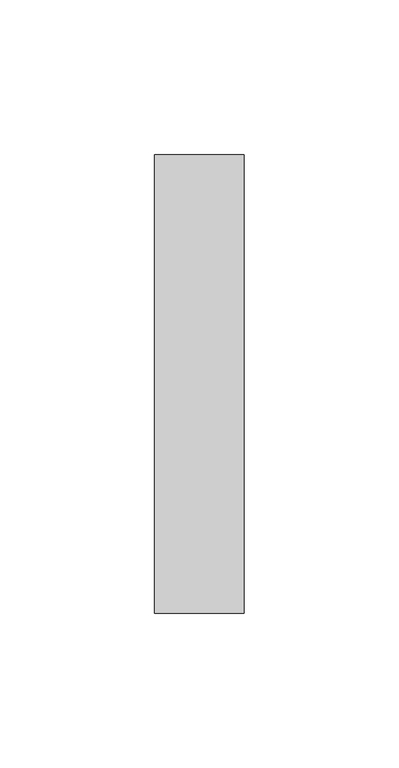
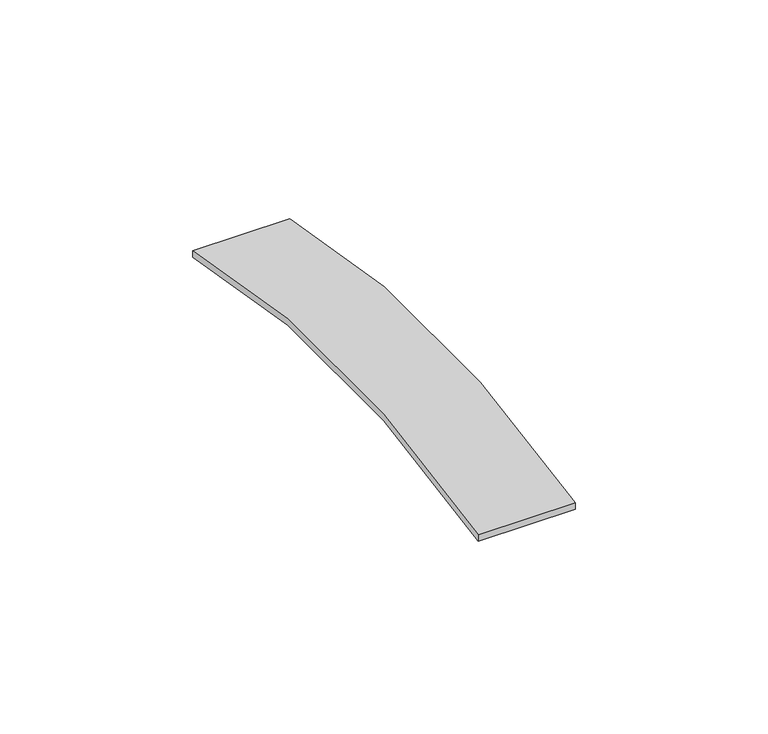
"""IFC4 building model written with IfcOpenShell, lengths in millimetres: proxy geometry, TN_ПВС 125-82_Защитная решетка : TN_ПВС 125-82_Защитная решетка."""

import ifcopenshell
import ifcopenshell.guid

model = None  # the IFC model being written
_history = None  # IfcOwnerHistory: only IFC2X3 demands one
_inside = {}  # id of a spatial element -> (the spatial element, [elements in it])
_under = {}  # id of a project, library or spatial element -> (it, [spatial elements below it])
_declared = {}  # id of a project -> (the project, [libraries it declares])
_typed = {}  # id of a type object -> (the type object, [elements of that type])
_made_of = {}  # id of a material, layer set ... -> (it, [elements and type objects made of it])


def new_model(schema):
    """Start an empty IFC model of exactly this schema.

    Asked for "IFC4X3", IfcOpenShell would pick the latest addendum, in which some entities
    have other attributes; the version numbers below select the first issue.
    IFC2X3 requires an IfcOwnerHistory on every rooted entity: one is made here for all.
    """
    global model, _history
    if schema == "IFC4X3":
        model = ifcopenshell.file(schema_version=(4, 3, 0, 0))
    else:
        model = ifcopenshell.file(schema=schema)
    _inside.clear()
    _under.clear()
    _declared.clear()
    _typed.clear()
    _made_of.clear()
    _history = None
    if model.schema == "IFC2X3":
        org = make("IfcOrganization", Name="unknown")
        user = make(
            "IfcPersonAndOrganization",
            ThePerson=make("IfcPerson", FamilyName="unknown"),
            TheOrganization=org,
        )
        app = make(
            "IfcApplication",
            ApplicationDeveloper=org,
            Version="unknown",
            ApplicationFullName="unknown",
            ApplicationIdentifier="unknown",
        )
        _history = make(
            "IfcOwnerHistory",
            OwningUser=user,
            OwningApplication=app,
            ChangeAction="ADDED",
            CreationDate=0,
        )
    return model


def make(cls, **values):
    """One entity of the class cls with the attributes given. An attribute that is None is left unset."""
    return model.create_entity(
        cls, **{name: value for name, value in values.items() if value is not None}
    )


def rooted(cls, **values):
    """An entity with a GlobalId (a new one), such as an element, a storey or a relation."""
    return make(cls, GlobalId=ifcopenshell.guid.new(), OwnerHistory=_history, **values)


def si_unit(unit_type, name, prefix=None):
    """IfcSIUnit, for example si_unit("LENGTHUNIT", "METRE", prefix="MILLI")."""
    return make("IfcSIUnit", UnitType=unit_type, Prefix=prefix, Name=name)


def assignment(units):
    """IfcUnitAssignment: the units of a project."""
    return None if units is None else make("IfcUnitAssignment", Units=units)


def point(xyz):
    """IfcCartesianPoint."""
    return None if xyz is None else make("IfcCartesianPoint", Coordinates=xyz)


def direction(xyz):
    """IfcDirection."""
    return None if xyz is None else make("IfcDirection", DirectionRatios=xyz)


def frame(location, z_axis=None, x_axis=None):
    """IfcAxis2Placement3D, a coordinate frame: its origin and axes. An axis left out is left unset."""
    return make(
        "IfcAxis2Placement3D",
        Location=point(location),
        Axis=direction(z_axis),
        RefDirection=direction(x_axis),
    )


def frame_2d(location, x_axis=None):
    """IfcAxis2Placement2D, a coordinate frame in the plane: its origin and x axis."""
    return make(
        "IfcAxis2Placement2D", Location=point(location), RefDirection=direction(x_axis)
    )


def origin():
    """The frame at (0, 0, 0) with its axes left unset."""
    return frame((0.0, 0.0, 0.0))


def place(relative_to, where):
    """IfcLocalPlacement: puts the frame where relative to a parent placement (None: the world)."""
    return make(
        "IfcLocalPlacement", PlacementRelTo=relative_to, RelativePlacement=where
    )


def context(
    kind, dimensions, precision=None, world=None, true_north=None, identifier=None
):
    """IfcGeometricRepresentationContext, for example the 3D "Model" context."""
    return make(
        "IfcGeometricRepresentationContext",
        ContextIdentifier=identifier,
        ContextType=kind,
        CoordinateSpaceDimension=dimensions,
        Precision=precision,
        WorldCoordinateSystem=world,
        TrueNorth=true_north,
    )


def project(units=None, contexts=None):
    """IfcProject with its units and contexts."""
    return rooted(
        "IfcProject",
        Name="project",
        RepresentationContexts=contexts,
        UnitsInContext=assignment(units),
    )


def spatial(cls, under=None, at=None, **own):
    """A site, building, storey or space (cls), placed at a placement, below another one or the project."""
    s = rooted(cls, ObjectPlacement=at, **own)
    if under is not None:
        _under.setdefault(under.id(), (under, []))[1].append(s)
    return s


def polyline(points):
    """IfcPolyline through the points."""
    return make("IfcPolyline", Points=[point(p) for p in points])


def circle_curve(where, radius):
    """IfcCircle in the frame where."""
    return make("IfcCircle", Position=where, Radius=radius)


def trimmed(basis, trim1, trim2, sense, master):
    """IfcTrimmedCurve: the piece of a basis curve between two trims."""
    return make(
        "IfcTrimmedCurve",
        BasisCurve=basis,
        Trim1=trim1,
        Trim2=trim2,
        SenseAgreement=sense,
        MasterRepresentation=master,
    )


def segment(curve, same_sense, transition):
    """IfcCompositeCurveSegment."""
    return make(
        "IfcCompositeCurveSegment",
        Transition=transition,
        SameSense=same_sense,
        ParentCurve=curve,
    )


def composite_curve(segments, self_intersect=None):
    """IfcCompositeCurve: segments joined end to end."""
    return make("IfcCompositeCurve", Segments=segments, SelfIntersect=self_intersect)


def outline(outer, holes=None, kind="AREA"):
    """IfcArbitraryClosedProfileDef: a profile drawn as a closed curve; with holes, ...WithVoids."""
    if holes is None:
        return make("IfcArbitraryClosedProfileDef", ProfileType=kind, OuterCurve=outer)
    return make(
        "IfcArbitraryProfileDefWithVoids",
        ProfileType=kind,
        OuterCurve=outer,
        InnerCurves=holes,
    )


def extrude(swept, where, along, depth):
    """IfcExtrudedAreaSolid: the profile swept, set in the frame where, extruded along a direction by depth."""
    return make(
        "IfcExtrudedAreaSolid",
        SweptArea=swept,
        Position=where,
        ExtrudedDirection=direction(along),
        Depth=depth,
    )


def shape(context_of_items, identifier, shape_type, items):
    """IfcShapeRepresentation: the items that make up one representation, for example the "Body"."""
    return make(
        "IfcShapeRepresentation",
        ContextOfItems=context_of_items,
        RepresentationIdentifier=identifier,
        RepresentationType=shape_type,
        Items=items,
    )


def source(mapping_origin, context_of_items, identifier, shape_type, items):
    """IfcRepresentationMap: a shape defined once, which mapped items show again and again."""
    return make(
        "IfcRepresentationMap",
        MappingOrigin=mapping_origin,
        MappedRepresentation=shape(context_of_items, identifier, shape_type, items),
    )


def transform(
    local_origin,
    x_axis=None,
    y_axis=None,
    z_axis=None,
    scale=None,
    scale2=None,
    scale3=None,
    uniform=True,
):
    """IfcCartesianTransformationOperator3D, or its non-uniform kind. x_axis, y_axis, z_axis: its Axis1, 2, 3."""
    if uniform:
        return make(
            "IfcCartesianTransformationOperator3D",
            Axis1=direction(x_axis),
            Axis2=direction(y_axis),
            LocalOrigin=point(local_origin),
            Scale=scale,
            Axis3=direction(z_axis),
        )
    return make(
        "IfcCartesianTransformationOperator3DnonUniform",
        Axis1=direction(x_axis),
        Axis2=direction(y_axis),
        LocalOrigin=point(local_origin),
        Scale=scale,
        Axis3=direction(z_axis),
        Scale2=scale2,
        Scale3=scale3,
    )


def mapped(mapping_source, mapping_target):
    """IfcMappedItem: shows the shape of a source again, moved by a transform."""
    return make(
        "IfcMappedItem", MappingSource=mapping_source, MappingTarget=mapping_target
    )


def made_of(thing, what):
    """Note that an element or type object is made of a material, layer set ...; save() writes the relation."""
    if what is not None:
        _made_of.setdefault(what.id(), (what, []))[1].append(thing)
    return thing


def element(
    cls,
    number,
    at=None,
    inside=None,
    cuts=None,
    type_object=None,
    material=None,
    context=None,
    identifier="Body",
    shape_type=None,
    held_by="IfcProductDefinitionShape",
    body=None,
    shapes=None,
    **own,
):
    """One element of the class cls, such as IfcWall. Its Tag is "e" and its number.

    at: its placement. inside: the storey or other place that contains it. cuts: it is an
    opening in that element (IfcRelVoidsElement). A single representation is given by context,
    identifier, shape_type and body (its items); several are given by shapes. held_by: the class
    of the entity that holds the representations. save() writes the other relations.
    """
    e = rooted(cls, Tag="e%d" % number, ObjectPlacement=at, **own)
    if body is not None:
        shapes = [shape(context, identifier, shape_type, body)]
    if shapes is not None:
        e.Representation = make(held_by, Representations=shapes)
    if inside is not None:
        _inside.setdefault(inside.id(), (inside, []))[1].append(e)
    if cuts is not None:
        rooted(
            "IfcRelVoidsElement", RelatingBuildingElement=cuts, RelatedOpeningElement=e
        )
    if type_object is not None:
        _typed.setdefault(type_object.id(), (type_object, []))[1].append(e)
    return made_of(e, material)


def aggregate(whole, parts):
    """IfcRelAggregates: a whole, such as a stair, and the parts it consists of."""
    return rooted("IfcRelAggregates", RelatingObject=whole, RelatedObjects=parts)


def save(model, path):
    """Write the relations noted so far, then the file.

    IfcRelAggregates (storeys below a building ...), IfcRelContainedInSpatialStructure (elements
    in a storey), IfcRelDefinesByType, IfcRelAssociatesMaterial and IfcRelDeclares: one each for
    every whole, place, type object, material and project.
    """
    for whole, parts in _under.values():
        aggregate(whole, parts)
    for where, things in _inside.values():
        rooted(
            "IfcRelContainedInSpatialStructure",
            RelatedElements=things,
            RelatingStructure=where,
        )
    for kind, things in _typed.values():
        rooted("IfcRelDefinesByType", RelatedObjects=things, RelatingType=kind)
    for what, things in _made_of.values():
        rooted("IfcRelAssociatesMaterial", RelatedObjects=things, RelatingMaterial=what)
    for by, libraries in _declared.values():
        rooted("IfcRelDeclares", RelatingContext=by, RelatedDefinitions=libraries)
    model.write(path)


def generic_models_660134d5(model_context):
    return source(origin(), model_context, "Body", "SweptSolid", [
        extrude(outline(composite_curve([segment(polyline([(-74.1, -0.0644007), (-74.1, 2.0)]), True, "CONTINUOUS"), segment(trimmed(circle_curve(frame_2d((0.0, -288.7046439)), 300.0), [point((-74.1, 2.0))], [point((74.1, 2.0))], False, "CARTESIAN"), True, "CONTINUOUS"), segment(polyline([(74.1, 2.0), (74.1, -0.0644007)]), True, "CONTINUOUS"), segment(trimmed(circle_curve(frame_2d((0.0, -288.7046439)), 298.0), [point((74.1, -0.0644007))], [point((-74.1, -0.0644007))], True, "CARTESIAN"), True, "CONTINUOUS")], self_intersect=False)), frame((0.0, 0.0, 0.0), z_axis=(1.0, 0.0, 0.0), x_axis=(0.0, 1.0, 0.0)), (0.0, 0.0, 1.0), 29.0),
    ])


if __name__ == "__main__":
    model = new_model("IFC4")
    model_context = context("Model", 3, world=origin())
    ifc_project = project(units=[si_unit("LENGTHUNIT", "METRE", prefix="MILLI")], contexts=[model_context])
    site = spatial("IfcSite", under=ifc_project)
    building = spatial("IfcBuilding", under=site)
    placement = place(None, origin())
    generic_models_shape = generic_models_660134d5(model_context)
    element("IfcBuildingElementProxy", 1, Name="TN_ПВС 125-82_Защитная решетка : TN_ПВС 125-82_Защитная решетка", ObjectType="TN_ПВС 125-82_Защитная решетка : TN_ПВС 125-82_Защитная решетка", at=placement, inside=building, context=model_context, shape_type="MappedRepresentation", body=[
        mapped(generic_models_shape, transform((0.0, 0.0, 0.0), x_axis=(1.0, 0.0, 0.0), y_axis=(0.0, 1.0, 0.0), z_axis=(0.0, 0.0, 1.0))),
    ])
    save(model, "model.ifc")

# Revit data of these elements
# Type "TN_ПВС 125-82_Защитная решетка : TN_ПВС 125-82_Защитная решетка"
#   Description = "Служит для предотвращения засора водосточной системы. Не пропускает в желоб листья и прочий крупный\r\nмусор"
#   Manufacturer = "ТехноНИКОЛЬ"
#   Model = "Комплектующие к водосточным системам"
#   URL = "https://tn-vodostok.ru/catalog/pvh/"
#   ADSK_Обозначение = "ТехноНИКОЛЬ"
#   ADSK_Наименование краткое = "Решетка"
#   ADSK_Наименование = "Защитная решетка"
#   ADSK_Масса_Текст = ""
#   ADSK_Марка = ""
#   ADSK_Код изделия = ""
#   ADSK_Завод-изготовитель = "ТехноНИКОЛЬ"
#   ADSK_Единица измерения = "п.м."
#   ADSK_Группирование = "Комплектующие к водосточным системам"
#   ADSK_URL страницы изделия = "https://tn-vodostok.ru/catalog/pvh/"
#   ADSK_URL документации изделия = "https://tn-vodostok.ru/upload/iblock/c42/c427963cb77eb5c3c51f0cfb870e9e52.pdf"
#   ADSK_Размер_Длина [instance default] = 500 mm
#   ADSK_Количество [instance default] = 0.5
#   ADSK_Материал [instance default] = TN_Пластик_Решетка_Коричневый_RAL8019
#   Default Elevation = 0
# Element 1 (IfcBuildingElementProxy, "TN_ПВС 125-82_Защитная решетка : TN_ПВС 125-82_Защитная решетка")
#   ADSK_Размер_Длина = 29 mm
#   ADSK_Количество = 0.029
#   Materials on its faces: "TN_Пластик_Решетка_Коричневый_RAL8019"
# Materials
#   "TN_Пластик_Решетка_Коричневый_RAL8019": class "Типовые", colour RGB 61 54 53, transparency 0.25, Cost = 0
